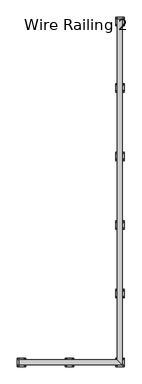
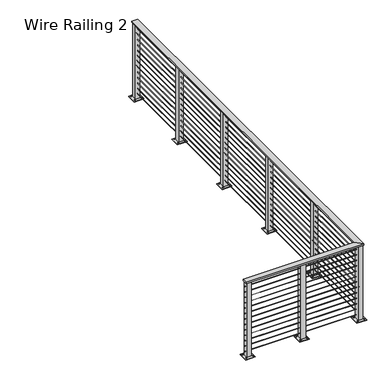
"""IFC4 building model written with IfcOpenShell, lengths in millimetres: railing geometry, Wire Railing 2."""

from ifc_helpers import new_model, si_unit, point, frame, frame_2d, origin, place, context, project, spatial, polyline, circle_curve, ellipse_curve, trimmed, segment, composite_curve, outline, extrude, faceted_brep, source, transform, mapped, element, save
from ifc_brep_helpers import plane_surface, cylinder_surface, advanced_brep


def wire_railing_2_7f4d2c74(model_context):
    return source(origin(), model_context, "Body", "SolidModel", [
        faceted_brep([(21482.8370052, 7634.1103648, 3870.325), (21559.0370052, 7634.1103648, 3870.325), (21559.0370052, 7634.1103648, 3851.275), (21482.8370052, 7634.1103648, 3851.275), (21559.0370052, 2430.2853648, 3870.325), (21559.0370052, 2430.2853648, 3851.275), (21482.8370052, 2506.4853648, 3870.325), (20003.2870052, 2506.4853648, 3870.325), (20003.2870052, 2506.4853648, 3851.275), (20003.2870052, 2430.2853648, 3851.275), (20003.2870052, 2430.2853648, 3870.325), (21482.8370052, 2506.4853648, 3851.275)], [[[0, 1, 2, 3]], [[2, 1, 4, 5]], [[1, 0, 6, 4]], [[7, 8, 9, 10]], [[5, 4, 10, 9]], [[4, 6, 7, 10]], [[3, 2, 5, 11]], [[0, 3, 11, 6]], [[11, 5, 9, 8]], [[6, 11, 8, 7]]]),
        advanced_brep(
        [(21523.3182552, 7634.1103648, 3791.74375), (21518.5557552, 7634.1103648, 3791.74375), (20003.2870052, 2466.0041148, 3791.74375), (20003.2870052, 2470.7666148, 3791.74375), (21523.3182552, 2466.0041148, 3791.74375), (21518.5557552, 2470.7666148, 3791.74375)],
        [
            (0, 1, circle_curve(frame((21520.9370052, 7634.1103648, 3791.74375), z_axis=(0.0, 1.0, 0.0), x_axis=(-1.0, 0.0, 0.0)), 2.38125)),
            (1, 0, circle_curve(frame((21520.9370052, 7634.1103648, 3791.74375), z_axis=(0.0, 1.0, 0.0), x_axis=(-1.0, 0.0, 0.0)), 2.38125)),
            (2, 3, circle_curve(frame((20003.2870052, 2468.3853648, 3791.74375), z_axis=(-1.0, 0.0, 0.0), x_axis=(0.0, 1.0, 0.0)), 2.38125)),
            (3, 2, circle_curve(frame((20003.2870052, 2468.3853648, 3791.74375), z_axis=(-1.0, 0.0, 0.0), x_axis=(0.0, 1.0, 0.0)), 2.38125)),
            (0, 4),
            (4, 5, ellipse_curve(frame((21520.9370052, 2468.3853648, 3791.74375), z_axis=(0.7071067811865475, 0.7071067811865475, 0.0), x_axis=(-0.7071067811865474, 0.7071067811865476, 0.0)), 3.367596, 2.38125)),
            (5, 1),
            (5, 4, ellipse_curve(frame((21520.9370052, 2468.3853648, 3791.74375), z_axis=(0.7071067811865475, 0.7071067811865475, 0.0), x_axis=(-0.7071067811865474, 0.7071067811865476, 0.0)), 3.367596, 2.38125)),
            (4, 2),
            (3, 5),
        ],
        [
            plane_surface(frame((21520.9370052, 7634.1103648, 3794.125), z_axis=(0.0, 1.0, 0.0), x_axis=(0.0, 0.0, -1.0))),
            plane_surface(frame((20003.2870052, 2468.3853648, 3794.125), z_axis=(-1.0, 0.0, 0.0), x_axis=(0.0, -1.0, 0.0))),
            cylinder_surface(frame((21520.9370052, 7634.1103648, 3791.74375), z_axis=(0.0, 1.0, 0.0), x_axis=(-1.0, 0.0, 0.0)), 2.38125),
            cylinder_surface(frame((21520.9370052, 2468.3853648, 3791.74375), z_axis=(1.0, 0.0, 0.0), x_axis=(0.0, 1.0, 0.0)), 2.38125),
        ],
        [
            (0, [[1, 2]]),
            (1, [[3, 4]]),
            (2, [[-1, 5, 6, 7]]),
            (2, [[-2, -7, 8, -5]]),
            (3, [[-6, 9, -4, 10]]),
            (3, [[-8, -10, -3, -9]]),
        ],
    ),
        advanced_brep(
        [(21523.3182552, 7634.1103648, 3715.54375), (21518.5557552, 7634.1103648, 3715.54375), (21523.3182552, 2466.0041148, 3715.54375), (21518.5557552, 2470.7666148, 3715.54375), (20003.2870052, 2466.0041148, 3715.54375), (20003.2870052, 2470.7666148, 3715.54375)],
        [
            (0, 1, circle_curve(frame((21520.9370052, 7634.1103648, 3715.54375), z_axis=(0.0, 1.0, 0.0), x_axis=(-1.0, 0.0, 0.0)), 2.38125)),
            (1, 0, circle_curve(frame((21520.9370052, 7634.1103648, 3715.54375), z_axis=(0.0, 1.0, 0.0), x_axis=(-1.0, 0.0, 0.0)), 2.38125)),
            (0, 2),
            (2, 3, ellipse_curve(frame((21520.9370052, 2468.3853648, 3715.54375), z_axis=(0.7071067811865475, 0.7071067811865475, 0.0), x_axis=(-0.7071067811865474, 0.7071067811865476, 0.0)), 3.367596, 2.38125)),
            (3, 1),
            (3, 2, ellipse_curve(frame((21520.9370052, 2468.3853648, 3715.54375), z_axis=(0.7071067811865475, 0.7071067811865475, 0.0), x_axis=(-0.7071067811865474, 0.7071067811865476, 0.0)), 3.367596, 2.38125)),
            (4, 5, circle_curve(frame((20003.2870052, 2468.3853648, 3715.54375), z_axis=(-1.0, 0.0, 0.0), x_axis=(0.0, 1.0, 0.0)), 2.38125)),
            (5, 4, circle_curve(frame((20003.2870052, 2468.3853648, 3715.54375), z_axis=(-1.0, 0.0, 0.0), x_axis=(0.0, 1.0, 0.0)), 2.38125)),
            (2, 4),
            (5, 3),
        ],
        [
            plane_surface(frame((21520.9370052, 7634.1103648, 3717.925), z_axis=(0.0, 1.0, 0.0), x_axis=(0.0, 0.0, -1.0))),
            cylinder_surface(frame((21520.9370052, 7634.1103648, 3715.54375), z_axis=(0.0, 1.0, 0.0), x_axis=(-1.0, 0.0, 0.0)), 2.38125),
            plane_surface(frame((20003.2870052, 2468.3853648, 3717.925), z_axis=(-1.0, 0.0, 0.0), x_axis=(0.0, -1.0, 0.0))),
            cylinder_surface(frame((21520.9370052, 2468.3853648, 3715.54375), z_axis=(1.0, 0.0, 0.0), x_axis=(0.0, 1.0, 0.0)), 2.38125),
        ],
        [
            (0, [[1, 2]]),
            (1, [[-1, 3, 4, 5]]),
            (1, [[-2, -5, 6, -3]]),
            (2, [[7, 8]]),
            (3, [[-4, 9, -8, 10]]),
            (3, [[-6, -10, -7, -9]]),
        ],
    ),
        advanced_brep(
        [(21523.3182552, 7634.1103648, 3639.34375), (21518.5557552, 7634.1103648, 3639.34375), (21523.3182552, 2466.0041148, 3639.34375), (21518.5557552, 2470.7666148, 3639.34375), (20003.2870052, 2466.0041148, 3639.34375), (20003.2870052, 2470.7666148, 3639.34375)],
        [
            (0, 1, circle_curve(frame((21520.9370052, 7634.1103648, 3639.34375), z_axis=(0.0, 1.0, 0.0), x_axis=(-1.0, 0.0, 0.0)), 2.38125)),
            (1, 0, circle_curve(frame((21520.9370052, 7634.1103648, 3639.34375), z_axis=(0.0, 1.0, 0.0), x_axis=(-1.0, 0.0, 0.0)), 2.38125)),
            (0, 2),
            (2, 3, ellipse_curve(frame((21520.9370052, 2468.3853648, 3639.34375), z_axis=(0.7071067811865475, 0.7071067811865475, 0.0), x_axis=(-0.7071067811865474, 0.7071067811865476, 0.0)), 3.367596, 2.38125)),
            (3, 1),
            (3, 2, ellipse_curve(frame((21520.9370052, 2468.3853648, 3639.34375), z_axis=(0.7071067811865475, 0.7071067811865475, 0.0), x_axis=(-0.7071067811865474, 0.7071067811865476, 0.0)), 3.367596, 2.38125)),
            (4, 5, circle_curve(frame((20003.2870052, 2468.3853648, 3639.34375), z_axis=(-1.0, 0.0, 0.0), x_axis=(0.0, 1.0, 0.0)), 2.38125)),
            (5, 4, circle_curve(frame((20003.2870052, 2468.3853648, 3639.34375), z_axis=(-1.0, 0.0, 0.0), x_axis=(0.0, 1.0, 0.0)), 2.38125)),
            (2, 4),
            (5, 3),
        ],
        [
            plane_surface(frame((21520.9370052, 7634.1103648, 3641.725), z_axis=(0.0, 1.0, 0.0), x_axis=(0.0, 0.0, -1.0))),
            cylinder_surface(frame((21520.9370052, 7634.1103648, 3639.34375), z_axis=(0.0, 1.0, 0.0), x_axis=(-1.0, 0.0, 0.0)), 2.38125),
            plane_surface(frame((20003.2870052, 2468.3853648, 3641.725), z_axis=(-1.0, 0.0, 0.0), x_axis=(0.0, -1.0, 0.0))),
            cylinder_surface(frame((21520.9370052, 2468.3853648, 3639.34375), z_axis=(1.0, 0.0, 0.0), x_axis=(0.0, 1.0, 0.0)), 2.38125),
        ],
        [
            (0, [[1, 2]]),
            (1, [[-1, 3, 4, 5]]),
            (1, [[-2, -5, 6, -3]]),
            (2, [[7, 8]]),
            (3, [[-4, 9, -8, 10]]),
            (3, [[-6, -10, -7, -9]]),
        ],
    ),
        advanced_brep(
        [(21523.3182552, 7634.1103648, 3563.14375), (21518.5557552, 7634.1103648, 3563.14375), (21523.3182552, 2466.0041148, 3563.14375), (21518.5557552, 2470.7666148, 3563.14375), (20003.2870052, 2466.0041148, 3563.14375), (20003.2870052, 2470.7666148, 3563.14375)],
        [
            (0, 1, circle_curve(frame((21520.9370052, 7634.1103648, 3563.14375), z_axis=(0.0, 1.0, 0.0), x_axis=(-1.0, 0.0, 0.0)), 2.38125)),
            (1, 0, circle_curve(frame((21520.9370052, 7634.1103648, 3563.14375), z_axis=(0.0, 1.0, 0.0), x_axis=(-1.0, 0.0, 0.0)), 2.38125)),
            (0, 2),
            (2, 3, ellipse_curve(frame((21520.9370052, 2468.3853648, 3563.14375), z_axis=(0.7071067811865475, 0.7071067811865475, 0.0), x_axis=(-0.7071067811865474, 0.7071067811865476, 0.0)), 3.367596, 2.38125)),
            (3, 1),
            (3, 2, ellipse_curve(frame((21520.9370052, 2468.3853648, 3563.14375), z_axis=(0.7071067811865475, 0.7071067811865475, 0.0), x_axis=(-0.7071067811865474, 0.7071067811865476, 0.0)), 3.367596, 2.38125)),
            (4, 5, circle_curve(frame((20003.2870052, 2468.3853648, 3563.14375), z_axis=(-1.0, 0.0, 0.0), x_axis=(0.0, 1.0, 0.0)), 2.38125)),
            (5, 4, circle_curve(frame((20003.2870052, 2468.3853648, 3563.14375), z_axis=(-1.0, 0.0, 0.0), x_axis=(0.0, 1.0, 0.0)), 2.38125)),
            (2, 4),
            (5, 3),
        ],
        [
            plane_surface(frame((21520.9370052, 7634.1103648, 3565.525), z_axis=(0.0, 1.0, 0.0), x_axis=(0.0, 0.0, -1.0))),
            cylinder_surface(frame((21520.9370052, 7634.1103648, 3563.14375), z_axis=(0.0, 1.0, 0.0), x_axis=(-1.0, 0.0, 0.0)), 2.38125),
            plane_surface(frame((20003.2870052, 2468.3853648, 3565.525), z_axis=(-1.0, 0.0, 0.0), x_axis=(0.0, -1.0, 0.0))),
            cylinder_surface(frame((21520.9370052, 2468.3853648, 3563.14375), z_axis=(1.0, 0.0, 0.0), x_axis=(0.0, 1.0, 0.0)), 2.38125),
        ],
        [
            (0, [[1, 2]]),
            (1, [[-1, 3, 4, 5]]),
            (1, [[-2, -5, 6, -3]]),
            (2, [[7, 8]]),
            (3, [[-4, 9, -8, 10]]),
            (3, [[-6, -10, -7, -9]]),
        ],
    ),
        advanced_brep(
        [(21523.3182552, 7634.1103648, 3486.94375), (21518.5557552, 7634.1103648, 3486.94375), (21523.3182552, 2466.0041148, 3486.94375), (21518.5557552, 2470.7666148, 3486.94375), (20003.2870052, 2466.0041148, 3486.94375), (20003.2870052, 2470.7666148, 3486.94375)],
        [
            (0, 1, circle_curve(frame((21520.9370052, 7634.1103648, 3486.94375), z_axis=(0.0, 1.0, 0.0), x_axis=(-1.0, 0.0, 0.0)), 2.38125)),
            (1, 0, circle_curve(frame((21520.9370052, 7634.1103648, 3486.94375), z_axis=(0.0, 1.0, 0.0), x_axis=(-1.0, 0.0, 0.0)), 2.38125)),
            (0, 2),
            (2, 3, ellipse_curve(frame((21520.9370052, 2468.3853648, 3486.94375), z_axis=(0.7071067811865475, 0.7071067811865475, 0.0), x_axis=(-0.7071067811865474, 0.7071067811865476, 0.0)), 3.367596, 2.38125)),
            (3, 1),
            (3, 2, ellipse_curve(frame((21520.9370052, 2468.3853648, 3486.94375), z_axis=(0.7071067811865475, 0.7071067811865475, 0.0), x_axis=(-0.7071067811865474, 0.7071067811865476, 0.0)), 3.367596, 2.38125)),
            (4, 5, circle_curve(frame((20003.2870052, 2468.3853648, 3486.94375), z_axis=(-1.0, 0.0, 0.0), x_axis=(0.0, 1.0, 0.0)), 2.38125)),
            (5, 4, circle_curve(frame((20003.2870052, 2468.3853648, 3486.94375), z_axis=(-1.0, 0.0, 0.0), x_axis=(0.0, 1.0, 0.0)), 2.38125)),
            (2, 4),
            (5, 3),
        ],
        [
            plane_surface(frame((21520.9370052, 7634.1103648, 3489.325), z_axis=(0.0, 1.0, 0.0), x_axis=(0.0, 0.0, -1.0))),
            cylinder_surface(frame((21520.9370052, 7634.1103648, 3486.94375), z_axis=(0.0, 1.0, 0.0), x_axis=(-1.0, 0.0, 0.0)), 2.38125),
            plane_surface(frame((20003.2870052, 2468.3853648, 3489.325), z_axis=(-1.0, 0.0, 0.0), x_axis=(0.0, -1.0, 0.0))),
            cylinder_surface(frame((21520.9370052, 2468.3853648, 3486.94375), z_axis=(1.0, 0.0, 0.0), x_axis=(0.0, 1.0, 0.0)), 2.38125),
        ],
        [
            (0, [[1, 2]]),
            (1, [[-1, 3, 4, 5]]),
            (1, [[-2, -5, 6, -3]]),
            (2, [[7, 8]]),
            (3, [[-4, 9, -8, 10]]),
            (3, [[-6, -10, -7, -9]]),
        ],
    ),
        advanced_brep(
        [(21523.3182552, 7634.1103648, 3410.74375), (21518.5557552, 7634.1103648, 3410.74375), (21523.3182552, 2466.0041148, 3410.74375), (21518.5557552, 2470.7666148, 3410.74375), (20003.2870052, 2466.0041148, 3410.74375), (20003.2870052, 2470.7666148, 3410.74375)],
        [
            (0, 1, circle_curve(frame((21520.9370052, 7634.1103648, 3410.74375), z_axis=(0.0, 1.0, 0.0), x_axis=(-1.0, 0.0, 0.0)), 2.38125)),
            (1, 0, circle_curve(frame((21520.9370052, 7634.1103648, 3410.74375), z_axis=(0.0, 1.0, 0.0), x_axis=(-1.0, 0.0, 0.0)), 2.38125)),
            (0, 2),
            (2, 3, ellipse_curve(frame((21520.9370052, 2468.3853648, 3410.74375), z_axis=(0.7071067811865475, 0.7071067811865475, 0.0), x_axis=(-0.7071067811865474, 0.7071067811865476, 0.0)), 3.367596, 2.38125)),
            (3, 1),
            (3, 2, ellipse_curve(frame((21520.9370052, 2468.3853648, 3410.74375), z_axis=(0.7071067811865475, 0.7071067811865475, 0.0), x_axis=(-0.7071067811865474, 0.7071067811865476, 0.0)), 3.367596, 2.38125)),
            (4, 5, circle_curve(frame((20003.2870052, 2468.3853648, 3410.74375), z_axis=(-1.0, 0.0, 0.0), x_axis=(0.0, 1.0, 0.0)), 2.38125)),
            (5, 4, circle_curve(frame((20003.2870052, 2468.3853648, 3410.74375), z_axis=(-1.0, 0.0, 0.0), x_axis=(0.0, 1.0, 0.0)), 2.38125)),
            (2, 4),
            (5, 3),
        ],
        [
            plane_surface(frame((21520.9370052, 7634.1103648, 3413.125), z_axis=(0.0, 1.0, 0.0), x_axis=(0.0, 0.0, -1.0))),
            cylinder_surface(frame((21520.9370052, 7634.1103648, 3410.74375), z_axis=(0.0, 1.0, 0.0), x_axis=(-1.0, 0.0, 0.0)), 2.38125),
            plane_surface(frame((20003.2870052, 2468.3853648, 3413.125), z_axis=(-1.0, 0.0, 0.0), x_axis=(0.0, -1.0, 0.0))),
            cylinder_surface(frame((21520.9370052, 2468.3853648, 3410.74375), z_axis=(1.0, 0.0, 0.0), x_axis=(0.0, 1.0, 0.0)), 2.38125),
        ],
        [
            (0, [[1, 2]]),
            (1, [[-1, 3, 4, 5]]),
            (1, [[-2, -5, 6, -3]]),
            (2, [[7, 8]]),
            (3, [[-4, 9, -8, 10]]),
            (3, [[-6, -10, -7, -9]]),
        ],
    ),
        advanced_brep(
        [(21523.3182552, 7634.1103648, 3334.54375), (21518.5557552, 7634.1103648, 3334.54375), (21523.3182552, 2466.0041148, 3334.54375), (21518.5557552, 2470.7666148, 3334.54375), (20003.2870052, 2466.0041148, 3334.54375), (20003.2870052, 2470.7666148, 3334.54375)],
        [
            (0, 1, circle_curve(frame((21520.9370052, 7634.1103648, 3334.54375), z_axis=(0.0, 1.0, 0.0), x_axis=(-1.0, 0.0, 0.0)), 2.38125)),
            (1, 0, circle_curve(frame((21520.9370052, 7634.1103648, 3334.54375), z_axis=(0.0, 1.0, 0.0), x_axis=(-1.0, 0.0, 0.0)), 2.38125)),
            (0, 2),
            (2, 3, ellipse_curve(frame((21520.9370052, 2468.3853648, 3334.54375), z_axis=(0.7071067811865475, 0.7071067811865475, 0.0), x_axis=(-0.7071067811865474, 0.7071067811865476, 0.0)), 3.367596, 2.38125)),
            (3, 1),
            (3, 2, ellipse_curve(frame((21520.9370052, 2468.3853648, 3334.54375), z_axis=(0.7071067811865475, 0.7071067811865475, 0.0), x_axis=(-0.7071067811865474, 0.7071067811865476, 0.0)), 3.367596, 2.38125)),
            (4, 5, circle_curve(frame((20003.2870052, 2468.3853648, 3334.54375), z_axis=(-1.0, 0.0, 0.0), x_axis=(0.0, 1.0, 0.0)), 2.38125)),
            (5, 4, circle_curve(frame((20003.2870052, 2468.3853648, 3334.54375), z_axis=(-1.0, 0.0, 0.0), x_axis=(0.0, 1.0, 0.0)), 2.38125)),
            (2, 4),
            (5, 3),
        ],
        [
            plane_surface(frame((21520.9370052, 7634.1103648, 3336.925), z_axis=(0.0, 1.0, 0.0), x_axis=(0.0, 0.0, -1.0))),
            cylinder_surface(frame((21520.9370052, 7634.1103648, 3334.54375), z_axis=(0.0, 1.0, 0.0), x_axis=(-1.0, 0.0, 0.0)), 2.38125),
            plane_surface(frame((20003.2870052, 2468.3853648, 3336.925), z_axis=(-1.0, 0.0, 0.0), x_axis=(0.0, -1.0, 0.0))),
            cylinder_surface(frame((21520.9370052, 2468.3853648, 3334.54375), z_axis=(1.0, 0.0, 0.0), x_axis=(0.0, 1.0, 0.0)), 2.38125),
        ],
        [
            (0, [[1, 2]]),
            (1, [[-1, 3, 4, 5]]),
            (1, [[-2, -5, 6, -3]]),
            (2, [[7, 8]]),
            (3, [[-4, 9, -8, 10]]),
            (3, [[-6, -10, -7, -9]]),
        ],
    ),
        advanced_brep(
        [(21523.3182552, 7634.1103648, 3258.34375), (21518.5557552, 7634.1103648, 3258.34375), (21523.3182552, 2466.0041148, 3258.34375), (21518.5557552, 2470.7666148, 3258.34375), (20003.2870052, 2466.0041148, 3258.34375), (20003.2870052, 2470.7666148, 3258.34375)],
        [
            (0, 1, circle_curve(frame((21520.9370052, 7634.1103648, 3258.34375), z_axis=(0.0, 1.0, 0.0), x_axis=(-1.0, 0.0, 0.0)), 2.38125)),
            (1, 0, circle_curve(frame((21520.9370052, 7634.1103648, 3258.34375), z_axis=(0.0, 1.0, 0.0), x_axis=(-1.0, 0.0, 0.0)), 2.38125)),
            (0, 2),
            (2, 3, ellipse_curve(frame((21520.9370052, 2468.3853648, 3258.34375), z_axis=(0.7071067811865475, 0.7071067811865475, 0.0), x_axis=(-0.7071067811865474, 0.7071067811865476, 0.0)), 3.367596, 2.38125)),
            (3, 1),
            (3, 2, ellipse_curve(frame((21520.9370052, 2468.3853648, 3258.34375), z_axis=(0.7071067811865475, 0.7071067811865475, 0.0), x_axis=(-0.7071067811865474, 0.7071067811865476, 0.0)), 3.367596, 2.38125)),
            (4, 5, circle_curve(frame((20003.2870052, 2468.3853648, 3258.34375), z_axis=(-1.0, 0.0, 0.0), x_axis=(0.0, 1.0, 0.0)), 2.38125)),
            (5, 4, circle_curve(frame((20003.2870052, 2468.3853648, 3258.34375), z_axis=(-1.0, 0.0, 0.0), x_axis=(0.0, 1.0, 0.0)), 2.38125)),
            (2, 4),
            (5, 3),
        ],
        [
            plane_surface(frame((21520.9370052, 7634.1103648, 3260.725), z_axis=(0.0, 1.0, 0.0), x_axis=(0.0, 0.0, -1.0))),
            cylinder_surface(frame((21520.9370052, 7634.1103648, 3258.34375), z_axis=(0.0, 1.0, 0.0), x_axis=(-1.0, 0.0, 0.0)), 2.38125),
            plane_surface(frame((20003.2870052, 2468.3853648, 3260.725), z_axis=(-1.0, 0.0, 0.0), x_axis=(0.0, -1.0, 0.0))),
            cylinder_surface(frame((21520.9370052, 2468.3853648, 3258.34375), z_axis=(1.0, 0.0, 0.0), x_axis=(0.0, 1.0, 0.0)), 2.38125),
        ],
        [
            (0, [[1, 2]]),
            (1, [[-1, 3, 4, 5]]),
            (1, [[-2, -5, 6, -3]]),
            (2, [[7, 8]]),
            (3, [[-4, 9, -8, 10]]),
            (3, [[-6, -10, -7, -9]]),
        ],
    ),
        advanced_brep(
        [(21523.3182552, 7634.1103648, 3182.14375), (21518.5557552, 7634.1103648, 3182.14375), (21523.3182552, 2466.0041148, 3182.14375), (21518.5557552, 2470.7666148, 3182.14375), (20003.2870052, 2466.0041148, 3182.14375), (20003.2870052, 2470.7666148, 3182.14375)],
        [
            (0, 1, circle_curve(frame((21520.9370052, 7634.1103648, 3182.14375), z_axis=(0.0, 1.0, 0.0), x_axis=(-1.0, 0.0, 0.0)), 2.38125)),
            (1, 0, circle_curve(frame((21520.9370052, 7634.1103648, 3182.14375), z_axis=(0.0, 1.0, 0.0), x_axis=(-1.0, 0.0, 0.0)), 2.38125)),
            (0, 2),
            (2, 3, ellipse_curve(frame((21520.9370052, 2468.3853648, 3182.14375), z_axis=(0.7071067811865475, 0.7071067811865475, 0.0), x_axis=(-0.7071067811865474, 0.7071067811865476, 0.0)), 3.367596, 2.38125)),
            (3, 1),
            (3, 2, ellipse_curve(frame((21520.9370052, 2468.3853648, 3182.14375), z_axis=(0.7071067811865475, 0.7071067811865475, 0.0), x_axis=(-0.7071067811865474, 0.7071067811865476, 0.0)), 3.367596, 2.38125)),
            (4, 5, circle_curve(frame((20003.2870052, 2468.3853648, 3182.14375), z_axis=(-1.0, 0.0, 0.0), x_axis=(0.0, 1.0, 0.0)), 2.38125)),
            (5, 4, circle_curve(frame((20003.2870052, 2468.3853648, 3182.14375), z_axis=(-1.0, 0.0, 0.0), x_axis=(0.0, 1.0, 0.0)), 2.38125)),
            (2, 4),
            (5, 3),
        ],
        [
            plane_surface(frame((21520.9370052, 7634.1103648, 3184.525), z_axis=(0.0, 1.0, 0.0), x_axis=(0.0, 0.0, -1.0))),
            cylinder_surface(frame((21520.9370052, 7634.1103648, 3182.14375), z_axis=(0.0, 1.0, 0.0), x_axis=(-1.0, 0.0, 0.0)), 2.38125),
            plane_surface(frame((20003.2870052, 2468.3853648, 3184.525), z_axis=(-1.0, 0.0, 0.0), x_axis=(0.0, -1.0, 0.0))),
            cylinder_surface(frame((21520.9370052, 2468.3853648, 3182.14375), z_axis=(1.0, 0.0, 0.0), x_axis=(0.0, 1.0, 0.0)), 2.38125),
        ],
        [
            (0, [[1, 2]]),
            (1, [[-1, 3, 4, 5]]),
            (1, [[-2, -5, 6, -3]]),
            (2, [[7, 8]]),
            (3, [[-4, 9, -8, 10]]),
            (3, [[-6, -10, -7, -9]]),
        ],
    ),
        advanced_brep(
        [(21523.3182552, 7634.1103648, 3105.94375), (21518.5557552, 7634.1103648, 3105.94375), (21523.3182552, 2466.0041148, 3105.94375), (21518.5557552, 2470.7666148, 3105.94375), (20003.2870052, 2466.0041148, 3105.94375), (20003.2870052, 2470.7666148, 3105.94375)],
        [
            (0, 1, circle_curve(frame((21520.9370052, 7634.1103648, 3105.94375), z_axis=(0.0, 1.0, 0.0), x_axis=(-1.0, 0.0, 0.0)), 2.38125)),
            (1, 0, circle_curve(frame((21520.9370052, 7634.1103648, 3105.94375), z_axis=(0.0, 1.0, 0.0), x_axis=(-1.0, 0.0, 0.0)), 2.38125)),
            (0, 2),
            (2, 3, ellipse_curve(frame((21520.9370052, 2468.3853648, 3105.94375), z_axis=(0.7071067811865475, 0.7071067811865475, 0.0), x_axis=(-0.7071067811865474, 0.7071067811865476, 0.0)), 3.367596, 2.38125)),
            (3, 1),
            (3, 2, ellipse_curve(frame((21520.9370052, 2468.3853648, 3105.94375), z_axis=(0.7071067811865475, 0.7071067811865475, 0.0), x_axis=(-0.7071067811865474, 0.7071067811865476, 0.0)), 3.367596, 2.38125)),
            (4, 5, circle_curve(frame((20003.2870052, 2468.3853648, 3105.94375), z_axis=(-1.0, 0.0, 0.0), x_axis=(0.0, 1.0, 0.0)), 2.38125)),
            (5, 4, circle_curve(frame((20003.2870052, 2468.3853648, 3105.94375), z_axis=(-1.0, 0.0, 0.0), x_axis=(0.0, 1.0, 0.0)), 2.38125)),
            (2, 4),
            (5, 3),
        ],
        [
            plane_surface(frame((21520.9370052, 7634.1103648, 3108.325), z_axis=(0.0, 1.0, 0.0), x_axis=(0.0, 0.0, -1.0))),
            cylinder_surface(frame((21520.9370052, 7634.1103648, 3105.94375), z_axis=(0.0, 1.0, 0.0), x_axis=(-1.0, 0.0, 0.0)), 2.38125),
            plane_surface(frame((20003.2870052, 2468.3853648, 3108.325), z_axis=(-1.0, 0.0, 0.0), x_axis=(0.0, -1.0, 0.0))),
            cylinder_surface(frame((21520.9370052, 2468.3853648, 3105.94375), z_axis=(1.0, 0.0, 0.0), x_axis=(0.0, 1.0, 0.0)), 2.38125),
        ],
        [
            (0, [[1, 2]]),
            (1, [[-1, 3, 4, 5]]),
            (1, [[-2, -5, 6, -3]]),
            (2, [[7, 8]]),
            (3, [[-4, 9, -8, 10]]),
            (3, [[-6, -10, -7, -9]]),
        ],
    ),
        advanced_brep(
        [(21523.3182552, 7634.1103648, 3029.74375), (21518.5557552, 7634.1103648, 3029.74375), (21523.3182552, 2466.0041148, 3029.74375), (21518.5557552, 2470.7666148, 3029.74375), (20003.2870052, 2466.0041148, 3029.74375), (20003.2870052, 2470.7666148, 3029.74375)],
        [
            (0, 1, circle_curve(frame((21520.9370052, 7634.1103648, 3029.74375), z_axis=(0.0, 1.0, 0.0), x_axis=(-1.0, 0.0, 0.0)), 2.38125)),
            (1, 0, circle_curve(frame((21520.9370052, 7634.1103648, 3029.74375), z_axis=(0.0, 1.0, 0.0), x_axis=(-1.0, 0.0, 0.0)), 2.38125)),
            (0, 2),
            (2, 3, ellipse_curve(frame((21520.9370052, 2468.3853648, 3029.74375), z_axis=(0.7071067811865475, 0.7071067811865475, 0.0), x_axis=(-0.7071067811865474, 0.7071067811865476, 0.0)), 3.367596, 2.38125)),
            (3, 1),
            (3, 2, ellipse_curve(frame((21520.9370052, 2468.3853648, 3029.74375), z_axis=(0.7071067811865475, 0.7071067811865475, 0.0), x_axis=(-0.7071067811865474, 0.7071067811865476, 0.0)), 3.367596, 2.38125)),
            (4, 5, circle_curve(frame((20003.2870052, 2468.3853648, 3029.74375), z_axis=(-1.0, 0.0, 0.0), x_axis=(0.0, 1.0, 0.0)), 2.38125)),
            (5, 4, circle_curve(frame((20003.2870052, 2468.3853648, 3029.74375), z_axis=(-1.0, 0.0, 0.0), x_axis=(0.0, 1.0, 0.0)), 2.38125)),
            (2, 4),
            (5, 3),
        ],
        [
            plane_surface(frame((21520.9370052, 7634.1103648, 3032.125), z_axis=(0.0, 1.0, 0.0), x_axis=(0.0, 0.0, -1.0))),
            cylinder_surface(frame((21520.9370052, 7634.1103648, 3029.74375), z_axis=(0.0, 1.0, 0.0), x_axis=(-1.0, 0.0, 0.0)), 2.38125),
            plane_surface(frame((20003.2870052, 2468.3853648, 3032.125), z_axis=(-1.0, 0.0, 0.0), x_axis=(0.0, -1.0, 0.0))),
            cylinder_surface(frame((21520.9370052, 2468.3853648, 3029.74375), z_axis=(1.0, 0.0, 0.0), x_axis=(0.0, 1.0, 0.0)), 2.38125),
        ],
        [
            (0, [[1, 2]]),
            (1, [[-1, 3, 4, 5]]),
            (1, [[-2, -5, 6, -3]]),
            (2, [[7, 8]]),
            (3, [[-4, 9, -8, 10]]),
            (3, [[-6, -10, -7, -9]]),
        ],
    ),
        advanced_brep(
        [(21523.3182552, 7634.1103648, 2953.54375), (21518.5557552, 7634.1103648, 2953.54375), (21523.3182552, 2466.0041148, 2953.54375), (21518.5557552, 2470.7666148, 2953.54375), (20003.2870052, 2466.0041148, 2953.54375), (20003.2870052, 2470.7666148, 2953.54375)],
        [
            (0, 1, circle_curve(frame((21520.9370052, 7634.1103648, 2953.54375), z_axis=(0.0, 1.0, 0.0), x_axis=(-1.0, 0.0, 0.0)), 2.38125)),
            (1, 0, circle_curve(frame((21520.9370052, 7634.1103648, 2953.54375), z_axis=(0.0, 1.0, 0.0), x_axis=(-1.0, 0.0, 0.0)), 2.38125)),
            (0, 2),
            (2, 3, ellipse_curve(frame((21520.9370052, 2468.3853648, 2953.54375), z_axis=(0.7071067811865475, 0.7071067811865475, 0.0), x_axis=(-0.7071067811865474, 0.7071067811865476, 0.0)), 3.367596, 2.38125)),
            (3, 1),
            (3, 2, ellipse_curve(frame((21520.9370052, 2468.3853648, 2953.54375), z_axis=(0.7071067811865475, 0.7071067811865475, 0.0), x_axis=(-0.7071067811865474, 0.7071067811865476, 0.0)), 3.367596, 2.38125)),
            (4, 5, circle_curve(frame((20003.2870052, 2468.3853648, 2953.54375), z_axis=(-1.0, 0.0, 0.0), x_axis=(0.0, 1.0, 0.0)), 2.38125)),
            (5, 4, circle_curve(frame((20003.2870052, 2468.3853648, 2953.54375), z_axis=(-1.0, 0.0, 0.0), x_axis=(0.0, 1.0, 0.0)), 2.38125)),
            (2, 4),
            (5, 3),
        ],
        [
            plane_surface(frame((21520.9370052, 7634.1103648, 2955.925), z_axis=(0.0, 1.0, 0.0), x_axis=(0.0, 0.0, -1.0))),
            cylinder_surface(frame((21520.9370052, 7634.1103648, 2953.54375), z_axis=(0.0, 1.0, 0.0), x_axis=(-1.0, 0.0, 0.0)), 2.38125),
            plane_surface(frame((20003.2870052, 2468.3853648, 2955.925), z_axis=(-1.0, 0.0, 0.0), x_axis=(0.0, -1.0, 0.0))),
            cylinder_surface(frame((21520.9370052, 2468.3853648, 2953.54375), z_axis=(1.0, 0.0, 0.0), x_axis=(0.0, 1.0, 0.0)), 2.38125),
        ],
        [
            (0, [[1, 2]]),
            (1, [[-1, 3, 4, 5]]),
            (1, [[-2, -5, 6, -3]]),
            (2, [[7, 8]]),
            (3, [[-4, 9, -8, 10]]),
            (3, [[-6, -10, -7, -9]]),
        ],
    ),
        advanced_brep(
        [(21523.3182552, 7634.1103648, 2877.34375), (21518.5557552, 7634.1103648, 2877.34375), (21523.3182552, 2466.0041148, 2877.34375), (21518.5557552, 2470.7666148, 2877.34375), (20003.2870052, 2466.0041148, 2877.34375), (20003.2870052, 2470.7666148, 2877.34375)],
        [
            (0, 1, circle_curve(frame((21520.9370052, 7634.1103648, 2877.34375), z_axis=(0.0, 1.0, 0.0), x_axis=(-1.0, 0.0, 0.0)), 2.38125)),
            (1, 0, circle_curve(frame((21520.9370052, 7634.1103648, 2877.34375), z_axis=(0.0, 1.0, 0.0), x_axis=(-1.0, 0.0, 0.0)), 2.38125)),
            (0, 2),
            (2, 3, ellipse_curve(frame((21520.9370052, 2468.3853648, 2877.34375), z_axis=(0.7071067811865475, 0.7071067811865475, 0.0), x_axis=(-0.7071067811865474, 0.7071067811865476, 0.0)), 3.367596, 2.38125)),
            (3, 1),
            (3, 2, ellipse_curve(frame((21520.9370052, 2468.3853648, 2877.34375), z_axis=(0.7071067811865475, 0.7071067811865475, 0.0), x_axis=(-0.7071067811865474, 0.7071067811865476, 0.0)), 3.367596, 2.38125)),
            (4, 5, circle_curve(frame((20003.2870052, 2468.3853648, 2877.34375), z_axis=(-1.0, 0.0, 0.0), x_axis=(0.0, 1.0, 0.0)), 2.38125)),
            (5, 4, circle_curve(frame((20003.2870052, 2468.3853648, 2877.34375), z_axis=(-1.0, 0.0, 0.0), x_axis=(0.0, 1.0, 0.0)), 2.38125)),
            (2, 4),
            (5, 3),
        ],
        [
            plane_surface(frame((21520.9370052, 7634.1103648, 2879.725), z_axis=(0.0, 1.0, 0.0), x_axis=(0.0, 0.0, -1.0))),
            cylinder_surface(frame((21520.9370052, 7634.1103648, 2877.34375), z_axis=(0.0, 1.0, 0.0), x_axis=(-1.0, 0.0, 0.0)), 2.38125),
            plane_surface(frame((20003.2870052, 2468.3853648, 2879.725), z_axis=(-1.0, 0.0, 0.0), x_axis=(0.0, -1.0, 0.0))),
            cylinder_surface(frame((21520.9370052, 2468.3853648, 2877.34375), z_axis=(1.0, 0.0, 0.0), x_axis=(0.0, 1.0, 0.0)), 2.38125),
        ],
        [
            (0, [[1, 2]]),
            (1, [[-1, 3, 4, 5]]),
            (1, [[-2, -5, 6, -3]]),
            (2, [[7, 8]]),
            (3, [[-4, 9, -8, 10]]),
            (3, [[-6, -10, -7, -9]]),
        ],
    ),
        extrude(outline(composite_curve([segment(trimmed(circle_curve(frame_2d((20806.5620052, 2512.8353648)), 6.35), [point((20806.5620052, 2519.1853648))], [point((20806.5620052, 2506.4853648))], False, "CARTESIAN"), True, "CONTINUOUS"), segment(trimmed(circle_curve(frame_2d((20806.5620052, 2512.8353648)), 6.35), [point((20806.5620052, 2506.4853648))], [point((20806.5620052, 2519.1853648))], False, "CARTESIAN"), True, "CONTINUOUS")], self_intersect=False)), frame((0.0, 0.0, 2803.525), z_axis=(0.0, 0.0, 1.0), x_axis=(1.0, 0.0, 0.0)), (0.0, 0.0, 1.0), 12.7),
        extrude(outline(composite_curve([segment(trimmed(circle_curve(frame_2d((20806.5620052, 2423.9353648)), 6.35), [point((20806.5620052, 2430.2853648))], [point((20806.5620052, 2417.5853648))], False, "CARTESIAN"), True, "CONTINUOUS"), segment(trimmed(circle_curve(frame_2d((20806.5620052, 2423.9353648)), 6.35), [point((20806.5620052, 2417.5853648))], [point((20806.5620052, 2430.2853648))], False, "CARTESIAN"), True, "CONTINUOUS")], self_intersect=False)), frame((0.0, 0.0, 2803.525), z_axis=(0.0, 0.0, 1.0), x_axis=(1.0, 0.0, 0.0)), (0.0, 0.0, 1.0), 12.7),
        extrude(outline(composite_curve([segment(trimmed(circle_curve(frame_2d((20717.6620052, 2512.8353648)), 6.35), [point((20717.6620052, 2519.1853648))], [point((20717.6620052, 2506.4853648))], False, "CARTESIAN"), True, "CONTINUOUS"), segment(trimmed(circle_curve(frame_2d((20717.6620052, 2512.8353648)), 6.35), [point((20717.6620052, 2506.4853648))], [point((20717.6620052, 2519.1853648))], False, "CARTESIAN"), True, "CONTINUOUS")], self_intersect=False)), frame((0.0, 0.0, 2803.525), z_axis=(0.0, 0.0, 1.0), x_axis=(1.0, 0.0, 0.0)), (0.0, 0.0, 1.0), 12.7),
        extrude(outline(composite_curve([segment(trimmed(circle_curve(frame_2d((20717.6620052, 2423.9353648)), 6.35), [point((20717.6620052, 2430.2853648))], [point((20717.6620052, 2417.5853648))], False, "CARTESIAN"), True, "CONTINUOUS"), segment(trimmed(circle_curve(frame_2d((20717.6620052, 2423.9353648)), 6.35), [point((20717.6620052, 2417.5853648))], [point((20717.6620052, 2430.2853648))], False, "CARTESIAN"), True, "CONTINUOUS")], self_intersect=False)), frame((0.0, 0.0, 2803.525), z_axis=(0.0, 0.0, 1.0), x_axis=(1.0, 0.0, 0.0)), (0.0, 0.0, 1.0), 12.7),
        extrude(outline(polyline([(20825.6120052, 2404.8853648), (20698.6120052, 2404.8853648), (20698.6120052, 2531.8853648), (20825.6120052, 2531.8853648), (20825.6120052, 2404.8853648)])), frame((0.0, 0.0, 2803.525), z_axis=(0.0, 0.0, 1.0), x_axis=(1.0, 0.0, 0.0)), (0.0, 0.0, 1.0), 6.35),
        extrude(outline(polyline([(20792.2745052, 2438.2228648), (20731.9495052, 2438.2228648), (20731.9495052, 2498.5478648), (20792.2745052, 2498.5478648), (20792.2745052, 2438.2228648)]), holes=[polyline([(20785.9245052, 2444.5728648), (20785.9245052, 2492.1978648), (20738.2995052, 2492.1978648), (20738.2995052, 2444.5728648), (20785.9245052, 2444.5728648)])]), frame((0.0, 0.0, 2803.525), z_axis=(0.0, 0.0, 1.0), x_axis=(1.0, 0.0, 0.0)), (0.0, 0.0, 1.0), 1047.75),
        extrude(outline(composite_curve([segment(trimmed(circle_curve(frame_2d((21476.4870052, 3545.9803648)), 6.35), [point((21470.1370052, 3545.9803648))], [point((21482.8370052, 3545.9803648))], False, "CARTESIAN"), True, "CONTINUOUS"), segment(trimmed(circle_curve(frame_2d((21476.4870052, 3545.9803648)), 6.35), [point((21482.8370052, 3545.9803648))], [point((21470.1370052, 3545.9803648))], False, "CARTESIAN"), True, "CONTINUOUS")], self_intersect=False)), frame((0.0, 0.0, 2803.525), z_axis=(0.0, 0.0, 1.0), x_axis=(1.0, 0.0, 0.0)), (0.0, 0.0, 1.0), 12.7),
        extrude(outline(composite_curve([segment(trimmed(circle_curve(frame_2d((21565.3870052, 3545.9803648)), 6.35), [point((21559.0370052, 3545.9803648))], [point((21571.7370052, 3545.9803648))], False, "CARTESIAN"), True, "CONTINUOUS"), segment(trimmed(circle_curve(frame_2d((21565.3870052, 3545.9803648)), 6.35), [point((21571.7370052, 3545.9803648))], [point((21559.0370052, 3545.9803648))], False, "CARTESIAN"), True, "CONTINUOUS")], self_intersect=False)), frame((0.0, 0.0, 2803.525), z_axis=(0.0, 0.0, 1.0), x_axis=(1.0, 0.0, 0.0)), (0.0, 0.0, 1.0), 12.7),
        extrude(outline(composite_curve([segment(trimmed(circle_curve(frame_2d((21476.4870052, 3457.0803648)), 6.35), [point((21470.1370052, 3457.0803648))], [point((21482.8370052, 3457.0803648))], False, "CARTESIAN"), True, "CONTINUOUS"), segment(trimmed(circle_curve(frame_2d((21476.4870052, 3457.0803648)), 6.35), [point((21482.8370052, 3457.0803648))], [point((21470.1370052, 3457.0803648))], False, "CARTESIAN"), True, "CONTINUOUS")], self_intersect=False)), frame((0.0, 0.0, 2803.525), z_axis=(0.0, 0.0, 1.0), x_axis=(1.0, 0.0, 0.0)), (0.0, 0.0, 1.0), 12.7),
        extrude(outline(composite_curve([segment(trimmed(circle_curve(frame_2d((21565.3870052, 3457.0803648)), 6.35), [point((21559.0370052, 3457.0803648))], [point((21571.7370052, 3457.0803648))], False, "CARTESIAN"), True, "CONTINUOUS"), segment(trimmed(circle_curve(frame_2d((21565.3870052, 3457.0803648)), 6.35), [point((21571.7370052, 3457.0803648))], [point((21559.0370052, 3457.0803648))], False, "CARTESIAN"), True, "CONTINUOUS")], self_intersect=False)), frame((0.0, 0.0, 2803.525), z_axis=(0.0, 0.0, 1.0), x_axis=(1.0, 0.0, 0.0)), (0.0, 0.0, 1.0), 12.7),
        extrude(outline(polyline([(21584.4370052, 3565.0303648), (21584.4370052, 3438.0303648), (21457.4370052, 3438.0303648), (21457.4370052, 3565.0303648), (21584.4370052, 3565.0303648)])), frame((0.0, 0.0, 2803.525), z_axis=(0.0, 0.0, 1.0), x_axis=(1.0, 0.0, 0.0)), (0.0, 0.0, 1.0), 6.35),
        extrude(outline(polyline([(21551.0995052, 3531.6928648), (21551.0995052, 3471.3678648), (21490.7745052, 3471.3678648), (21490.7745052, 3531.6928648), (21551.0995052, 3531.6928648)]), holes=[polyline([(21544.7495052, 3525.3428648), (21497.1245052, 3525.3428648), (21497.1245052, 3477.7178648), (21544.7495052, 3477.7178648), (21544.7495052, 3525.3428648)])]), frame((0.0, 0.0, 2803.525), z_axis=(0.0, 0.0, 1.0), x_axis=(1.0, 0.0, 0.0)), (0.0, 0.0, 1.0), 1047.75),
        extrude(outline(composite_curve([segment(trimmed(circle_curve(frame_2d((21476.4870052, 4579.1253648)), 6.35), [point((21470.1370052, 4579.1253648))], [point((21482.8370052, 4579.1253648))], False, "CARTESIAN"), True, "CONTINUOUS"), segment(trimmed(circle_curve(frame_2d((21476.4870052, 4579.1253648)), 6.35), [point((21482.8370052, 4579.1253648))], [point((21470.1370052, 4579.1253648))], False, "CARTESIAN"), True, "CONTINUOUS")], self_intersect=False)), frame((0.0, 0.0, 2803.525), z_axis=(0.0, 0.0, 1.0), x_axis=(1.0, 0.0, 0.0)), (0.0, 0.0, 1.0), 12.7),
        extrude(outline(composite_curve([segment(trimmed(circle_curve(frame_2d((21565.3870052, 4579.1253648)), 6.35), [point((21559.0370052, 4579.1253648))], [point((21571.7370052, 4579.1253648))], False, "CARTESIAN"), True, "CONTINUOUS"), segment(trimmed(circle_curve(frame_2d((21565.3870052, 4579.1253648)), 6.35), [point((21571.7370052, 4579.1253648))], [point((21559.0370052, 4579.1253648))], False, "CARTESIAN"), True, "CONTINUOUS")], self_intersect=False)), frame((0.0, 0.0, 2803.525), z_axis=(0.0, 0.0, 1.0), x_axis=(1.0, 0.0, 0.0)), (0.0, 0.0, 1.0), 12.7),
        extrude(outline(composite_curve([segment(trimmed(circle_curve(frame_2d((21476.4870052, 4490.2253648)), 6.35), [point((21470.1370052, 4490.2253648))], [point((21482.8370052, 4490.2253648))], False, "CARTESIAN"), True, "CONTINUOUS"), segment(trimmed(circle_curve(frame_2d((21476.4870052, 4490.2253648)), 6.35), [point((21482.8370052, 4490.2253648))], [point((21470.1370052, 4490.2253648))], False, "CARTESIAN"), True, "CONTINUOUS")], self_intersect=False)), frame((0.0, 0.0, 2803.525), z_axis=(0.0, 0.0, 1.0), x_axis=(1.0, 0.0, 0.0)), (0.0, 0.0, 1.0), 12.7),
        extrude(outline(composite_curve([segment(trimmed(circle_curve(frame_2d((21565.3870052, 4490.2253648)), 6.35), [point((21559.0370052, 4490.2253648))], [point((21571.7370052, 4490.2253648))], False, "CARTESIAN"), True, "CONTINUOUS"), segment(trimmed(circle_curve(frame_2d((21565.3870052, 4490.2253648)), 6.35), [point((21571.7370052, 4490.2253648))], [point((21559.0370052, 4490.2253648))], False, "CARTESIAN"), True, "CONTINUOUS")], self_intersect=False)), frame((0.0, 0.0, 2803.525), z_axis=(0.0, 0.0, 1.0), x_axis=(1.0, 0.0, 0.0)), (0.0, 0.0, 1.0), 12.7),
        extrude(outline(polyline([(21584.4370052, 4598.1753648), (21584.4370052, 4471.1753648), (21457.4370052, 4471.1753648), (21457.4370052, 4598.1753648), (21584.4370052, 4598.1753648)])), frame((0.0, 0.0, 2803.525), z_axis=(0.0, 0.0, 1.0), x_axis=(1.0, 0.0, 0.0)), (0.0, 0.0, 1.0), 6.35),
        extrude(outline(polyline([(21551.0995052, 4564.8378648), (21551.0995052, 4504.5128648), (21490.7745052, 4504.5128648), (21490.7745052, 4564.8378648), (21551.0995052, 4564.8378648)]), holes=[polyline([(21544.7495052, 4558.4878648), (21497.1245052, 4558.4878648), (21497.1245052, 4510.8628648), (21544.7495052, 4510.8628648), (21544.7495052, 4558.4878648)])]), frame((0.0, 0.0, 2803.525), z_axis=(0.0, 0.0, 1.0), x_axis=(1.0, 0.0, 0.0)), (0.0, 0.0, 1.0), 1047.75),
        extrude(outline(composite_curve([segment(trimmed(circle_curve(frame_2d((21476.4870052, 5612.2703648)), 6.35), [point((21470.1370052, 5612.2703648))], [point((21482.8370052, 5612.2703648))], False, "CARTESIAN"), True, "CONTINUOUS"), segment(trimmed(circle_curve(frame_2d((21476.4870052, 5612.2703648)), 6.35), [point((21482.8370052, 5612.2703648))], [point((21470.1370052, 5612.2703648))], False, "CARTESIAN"), True, "CONTINUOUS")], self_intersect=False)), frame((0.0, 0.0, 2803.525), z_axis=(0.0, 0.0, 1.0), x_axis=(1.0, 0.0, 0.0)), (0.0, 0.0, 1.0), 12.7),
        extrude(outline(composite_curve([segment(trimmed(circle_curve(frame_2d((21565.3870052, 5612.2703648)), 6.35), [point((21559.0370052, 5612.2703648))], [point((21571.7370052, 5612.2703648))], False, "CARTESIAN"), True, "CONTINUOUS"), segment(trimmed(circle_curve(frame_2d((21565.3870052, 5612.2703648)), 6.35), [point((21571.7370052, 5612.2703648))], [point((21559.0370052, 5612.2703648))], False, "CARTESIAN"), True, "CONTINUOUS")], self_intersect=False)), frame((0.0, 0.0, 2803.525), z_axis=(0.0, 0.0, 1.0), x_axis=(1.0, 0.0, 0.0)), (0.0, 0.0, 1.0), 12.7),
        extrude(outline(composite_curve([segment(trimmed(circle_curve(frame_2d((21476.4870052, 5523.3703648)), 6.35), [point((21470.1370052, 5523.3703648))], [point((21482.8370052, 5523.3703648))], False, "CARTESIAN"), True, "CONTINUOUS"), segment(trimmed(circle_curve(frame_2d((21476.4870052, 5523.3703648)), 6.35), [point((21482.8370052, 5523.3703648))], [point((21470.1370052, 5523.3703648))], False, "CARTESIAN"), True, "CONTINUOUS")], self_intersect=False)), frame((0.0, 0.0, 2803.525), z_axis=(0.0, 0.0, 1.0), x_axis=(1.0, 0.0, 0.0)), (0.0, 0.0, 1.0), 12.7),
        extrude(outline(composite_curve([segment(trimmed(circle_curve(frame_2d((21565.3870052, 5523.3703648)), 6.35), [point((21559.0370052, 5523.3703648))], [point((21571.7370052, 5523.3703648))], False, "CARTESIAN"), True, "CONTINUOUS"), segment(trimmed(circle_curve(frame_2d((21565.3870052, 5523.3703648)), 6.35), [point((21571.7370052, 5523.3703648))], [point((21559.0370052, 5523.3703648))], False, "CARTESIAN"), True, "CONTINUOUS")], self_intersect=False)), frame((0.0, 0.0, 2803.525), z_axis=(0.0, 0.0, 1.0), x_axis=(1.0, 0.0, 0.0)), (0.0, 0.0, 1.0), 12.7),
        extrude(outline(polyline([(21584.4370052, 5631.3203648), (21584.4370052, 5504.3203648), (21457.4370052, 5504.3203648), (21457.4370052, 5631.3203648), (21584.4370052, 5631.3203648)])), frame((0.0, 0.0, 2803.525), z_axis=(0.0, 0.0, 1.0), x_axis=(1.0, 0.0, 0.0)), (0.0, 0.0, 1.0), 6.35),
        extrude(outline(polyline([(21551.0995052, 5597.9828648), (21551.0995052, 5537.6578648), (21490.7745052, 5537.6578648), (21490.7745052, 5597.9828648), (21551.0995052, 5597.9828648)]), holes=[polyline([(21544.7495052, 5591.6328648), (21497.1245052, 5591.6328648), (21497.1245052, 5544.0078648), (21544.7495052, 5544.0078648), (21544.7495052, 5591.6328648)])]), frame((0.0, 0.0, 2803.525), z_axis=(0.0, 0.0, 1.0), x_axis=(1.0, 0.0, 0.0)), (0.0, 0.0, 1.0), 1047.75),
        extrude(outline(composite_curve([segment(trimmed(circle_curve(frame_2d((21476.4870052, 6645.4153648)), 6.35), [point((21470.1370052, 6645.4153648))], [point((21482.8370052, 6645.4153648))], False, "CARTESIAN"), True, "CONTINUOUS"), segment(trimmed(circle_curve(frame_2d((21476.4870052, 6645.4153648)), 6.35), [point((21482.8370052, 6645.4153648))], [point((21470.1370052, 6645.4153648))], False, "CARTESIAN"), True, "CONTINUOUS")], self_intersect=False)), frame((0.0, 0.0, 2803.525), z_axis=(0.0, 0.0, 1.0), x_axis=(1.0, 0.0, 0.0)), (0.0, 0.0, 1.0), 12.7),
        extrude(outline(composite_curve([segment(trimmed(circle_curve(frame_2d((21565.3870052, 6645.4153648)), 6.35), [point((21559.0370052, 6645.4153648))], [point((21571.7370052, 6645.4153648))], False, "CARTESIAN"), True, "CONTINUOUS"), segment(trimmed(circle_curve(frame_2d((21565.3870052, 6645.4153648)), 6.35), [point((21571.7370052, 6645.4153648))], [point((21559.0370052, 6645.4153648))], False, "CARTESIAN"), True, "CONTINUOUS")], self_intersect=False)), frame((0.0, 0.0, 2803.525), z_axis=(0.0, 0.0, 1.0), x_axis=(1.0, 0.0, 0.0)), (0.0, 0.0, 1.0), 12.7),
        extrude(outline(composite_curve([segment(trimmed(circle_curve(frame_2d((21476.4870052, 6556.5153648)), 6.35), [point((21470.1370052, 6556.5153648))], [point((21482.8370052, 6556.5153648))], False, "CARTESIAN"), True, "CONTINUOUS"), segment(trimmed(circle_curve(frame_2d((21476.4870052, 6556.5153648)), 6.35), [point((21482.8370052, 6556.5153648))], [point((21470.1370052, 6556.5153648))], False, "CARTESIAN"), True, "CONTINUOUS")], self_intersect=False)), frame((0.0, 0.0, 2803.525), z_axis=(0.0, 0.0, 1.0), x_axis=(1.0, 0.0, 0.0)), (0.0, 0.0, 1.0), 12.7),
        extrude(outline(composite_curve([segment(trimmed(circle_curve(frame_2d((21565.3870052, 6556.5153648)), 6.35), [point((21559.0370052, 6556.5153648))], [point((21571.7370052, 6556.5153648))], False, "CARTESIAN"), True, "CONTINUOUS"), segment(trimmed(circle_curve(frame_2d((21565.3870052, 6556.5153648)), 6.35), [point((21571.7370052, 6556.5153648))], [point((21559.0370052, 6556.5153648))], False, "CARTESIAN"), True, "CONTINUOUS")], self_intersect=False)), frame((0.0, 0.0, 2803.525), z_axis=(0.0, 0.0, 1.0), x_axis=(1.0, 0.0, 0.0)), (0.0, 0.0, 1.0), 12.7),
        extrude(outline(polyline([(21584.4370052, 6664.4653648), (21584.4370052, 6537.4653648), (21457.4370052, 6537.4653648), (21457.4370052, 6664.4653648), (21584.4370052, 6664.4653648)])), frame((0.0, 0.0, 2803.525), z_axis=(0.0, 0.0, 1.0), x_axis=(1.0, 0.0, 0.0)), (0.0, 0.0, 1.0), 6.35),
        extrude(outline(polyline([(21551.0995052, 6631.1278648), (21551.0995052, 6570.8028648), (21490.7745052, 6570.8028648), (21490.7745052, 6631.1278648), (21551.0995052, 6631.1278648)]), holes=[polyline([(21544.7495052, 6624.7778648), (21497.1245052, 6624.7778648), (21497.1245052, 6577.1528648), (21544.7495052, 6577.1528648), (21544.7495052, 6624.7778648)])]), frame((0.0, 0.0, 2803.525), z_axis=(0.0, 0.0, 1.0), x_axis=(1.0, 0.0, 0.0)), (0.0, 0.0, 1.0), 1047.75),
        extrude(outline(composite_curve([segment(trimmed(circle_curve(frame_2d((21476.4870052, 2512.8353648)), 6.35), [point((21470.1370052, 2512.8353648))], [point((21482.8370052, 2512.8353648))], False, "CARTESIAN"), True, "CONTINUOUS"), segment(trimmed(circle_curve(frame_2d((21476.4870052, 2512.8353648)), 6.35), [point((21482.8370052, 2512.8353648))], [point((21470.1370052, 2512.8353648))], False, "CARTESIAN"), True, "CONTINUOUS")], self_intersect=False)), frame((0.0, 0.0, 2803.525), z_axis=(0.0, 0.0, 1.0), x_axis=(1.0, 0.0, 0.0)), (0.0, 0.0, 1.0), 12.7),
        extrude(outline(composite_curve([segment(trimmed(circle_curve(frame_2d((21565.3870052, 2512.8353648)), 6.35), [point((21559.0370052, 2512.8353648))], [point((21571.7370052, 2512.8353648))], False, "CARTESIAN"), True, "CONTINUOUS"), segment(trimmed(circle_curve(frame_2d((21565.3870052, 2512.8353648)), 6.35), [point((21571.7370052, 2512.8353648))], [point((21559.0370052, 2512.8353648))], False, "CARTESIAN"), True, "CONTINUOUS")], self_intersect=False)), frame((0.0, 0.0, 2803.525), z_axis=(0.0, 0.0, 1.0), x_axis=(1.0, 0.0, 0.0)), (0.0, 0.0, 1.0), 12.7),
        extrude(outline(composite_curve([segment(trimmed(circle_curve(frame_2d((21476.4870052, 2423.9353648)), 6.35), [point((21470.1370052, 2423.9353648))], [point((21482.8370052, 2423.9353648))], False, "CARTESIAN"), True, "CONTINUOUS"), segment(trimmed(circle_curve(frame_2d((21476.4870052, 2423.9353648)), 6.35), [point((21482.8370052, 2423.9353648))], [point((21470.1370052, 2423.9353648))], False, "CARTESIAN"), True, "CONTINUOUS")], self_intersect=False)), frame((0.0, 0.0, 2803.525), z_axis=(0.0, 0.0, 1.0), x_axis=(1.0, 0.0, 0.0)), (0.0, 0.0, 1.0), 12.7),
        extrude(outline(composite_curve([segment(trimmed(circle_curve(frame_2d((21565.3870052, 2423.9353648)), 6.35), [point((21559.0370052, 2423.9353648))], [point((21571.7370052, 2423.9353648))], False, "CARTESIAN"), True, "CONTINUOUS"), segment(trimmed(circle_curve(frame_2d((21565.3870052, 2423.9353648)), 6.35), [point((21571.7370052, 2423.9353648))], [point((21559.0370052, 2423.9353648))], False, "CARTESIAN"), True, "CONTINUOUS")], self_intersect=False)), frame((0.0, 0.0, 2803.525), z_axis=(0.0, 0.0, 1.0), x_axis=(1.0, 0.0, 0.0)), (0.0, 0.0, 1.0), 12.7),
        extrude(outline(polyline([(21584.4370052, 2531.8853648), (21584.4370052, 2404.8853648), (21457.4370052, 2404.8853648), (21457.4370052, 2531.8853648), (21584.4370052, 2531.8853648)])), frame((0.0, 0.0, 2803.525), z_axis=(0.0, 0.0, 1.0), x_axis=(1.0, 0.0, 0.0)), (0.0, 0.0, 1.0), 6.35),
        extrude(outline(polyline([(21551.0995052, 2498.5478648), (21551.0995052, 2438.2228648), (21490.7745052, 2438.2228648), (21490.7745052, 2498.5478648), (21551.0995052, 2498.5478648)]), holes=[polyline([(21544.7495052, 2492.1978648), (21497.1245052, 2492.1978648), (21497.1245052, 2444.5728648), (21544.7495052, 2444.5728648), (21544.7495052, 2492.1978648)])]), frame((0.0, 0.0, 2803.525), z_axis=(0.0, 0.0, 1.0), x_axis=(1.0, 0.0, 0.0)), (0.0, 0.0, 1.0), 1047.75),
        extrude(outline(composite_curve([segment(trimmed(circle_curve(frame_2d((20085.8370052, 2512.8353648)), 6.35), [point((20085.8370052, 2519.1853648))], [point((20085.8370052, 2506.4853648))], False, "CARTESIAN"), True, "CONTINUOUS"), segment(trimmed(circle_curve(frame_2d((20085.8370052, 2512.8353648)), 6.35), [point((20085.8370052, 2506.4853648))], [point((20085.8370052, 2519.1853648))], False, "CARTESIAN"), True, "CONTINUOUS")], self_intersect=False)), frame((0.0, 0.0, 2803.525), z_axis=(0.0, 0.0, 1.0), x_axis=(1.0, 0.0, 0.0)), (0.0, 0.0, 1.0), 12.7),
        extrude(outline(composite_curve([segment(trimmed(circle_curve(frame_2d((20085.8370052, 2423.9353648)), 6.35), [point((20085.8370052, 2430.2853648))], [point((20085.8370052, 2417.5853648))], False, "CARTESIAN"), True, "CONTINUOUS"), segment(trimmed(circle_curve(frame_2d((20085.8370052, 2423.9353648)), 6.35), [point((20085.8370052, 2417.5853648))], [point((20085.8370052, 2430.2853648))], False, "CARTESIAN"), True, "CONTINUOUS")], self_intersect=False)), frame((0.0, 0.0, 2803.525), z_axis=(0.0, 0.0, 1.0), x_axis=(1.0, 0.0, 0.0)), (0.0, 0.0, 1.0), 12.7),
        extrude(outline(composite_curve([segment(trimmed(circle_curve(frame_2d((19996.9370052, 2512.8353648)), 6.35), [point((19996.9370052, 2519.1853648))], [point((19996.9370052, 2506.4853648))], False, "CARTESIAN"), True, "CONTINUOUS"), segment(trimmed(circle_curve(frame_2d((19996.9370052, 2512.8353648)), 6.35), [point((19996.9370052, 2506.4853648))], [point((19996.9370052, 2519.1853648))], False, "CARTESIAN"), True, "CONTINUOUS")], self_intersect=False)), frame((0.0, 0.0, 2803.525), z_axis=(0.0, 0.0, 1.0), x_axis=(1.0, 0.0, 0.0)), (0.0, 0.0, 1.0), 12.7),
        extrude(outline(composite_curve([segment(trimmed(circle_curve(frame_2d((19996.9370052, 2423.9353648)), 6.35), [point((19996.9370052, 2430.2853648))], [point((19996.9370052, 2417.5853648))], False, "CARTESIAN"), True, "CONTINUOUS"), segment(trimmed(circle_curve(frame_2d((19996.9370052, 2423.9353648)), 6.35), [point((19996.9370052, 2417.5853648))], [point((19996.9370052, 2430.2853648))], False, "CARTESIAN"), True, "CONTINUOUS")], self_intersect=False)), frame((0.0, 0.0, 2803.525), z_axis=(0.0, 0.0, 1.0), x_axis=(1.0, 0.0, 0.0)), (0.0, 0.0, 1.0), 12.7),
        extrude(outline(polyline([(20104.8870052, 2404.8853648), (19977.8870052, 2404.8853648), (19977.8870052, 2531.8853648), (20104.8870052, 2531.8853648), (20104.8870052, 2404.8853648)])), frame((0.0, 0.0, 2803.525), z_axis=(0.0, 0.0, 1.0), x_axis=(1.0, 0.0, 0.0)), (0.0, 0.0, 1.0), 6.35),
        extrude(outline(polyline([(20071.5495052, 2438.2228648), (20011.2245052, 2438.2228648), (20011.2245052, 2498.5478648), (20071.5495052, 2498.5478648), (20071.5495052, 2438.2228648)]), holes=[polyline([(20065.1995052, 2444.5728648), (20065.1995052, 2492.1978648), (20017.5745052, 2492.1978648), (20017.5745052, 2444.5728648), (20065.1995052, 2444.5728648)])]), frame((0.0, 0.0, 2803.525), z_axis=(0.0, 0.0, 1.0), x_axis=(1.0, 0.0, 0.0)), (0.0, 0.0, 1.0), 1047.75),
        extrude(outline(composite_curve([segment(trimmed(circle_curve(frame_2d((21476.4870052, 7640.4603648)), 6.35), [point((21470.1370052, 7640.4603648))], [point((21482.8370052, 7640.4603648))], False, "CARTESIAN"), True, "CONTINUOUS"), segment(trimmed(circle_curve(frame_2d((21476.4870052, 7640.4603648)), 6.35), [point((21482.8370052, 7640.4603648))], [point((21470.1370052, 7640.4603648))], False, "CARTESIAN"), True, "CONTINUOUS")], self_intersect=False)), frame((0.0, 0.0, 2803.525), z_axis=(0.0, 0.0, 1.0), x_axis=(1.0, 0.0, 0.0)), (0.0, 0.0, 1.0), 12.7),
        extrude(outline(composite_curve([segment(trimmed(circle_curve(frame_2d((21565.3870052, 7640.4603648)), 6.35), [point((21559.0370052, 7640.4603648))], [point((21571.7370052, 7640.4603648))], False, "CARTESIAN"), True, "CONTINUOUS"), segment(trimmed(circle_curve(frame_2d((21565.3870052, 7640.4603648)), 6.35), [point((21571.7370052, 7640.4603648))], [point((21559.0370052, 7640.4603648))], False, "CARTESIAN"), True, "CONTINUOUS")], self_intersect=False)), frame((0.0, 0.0, 2803.525), z_axis=(0.0, 0.0, 1.0), x_axis=(1.0, 0.0, 0.0)), (0.0, 0.0, 1.0), 12.7),
        extrude(outline(composite_curve([segment(trimmed(circle_curve(frame_2d((21476.4870052, 7551.5603648)), 6.35), [point((21470.1370052, 7551.5603648))], [point((21482.8370052, 7551.5603648))], False, "CARTESIAN"), True, "CONTINUOUS"), segment(trimmed(circle_curve(frame_2d((21476.4870052, 7551.5603648)), 6.35), [point((21482.8370052, 7551.5603648))], [point((21470.1370052, 7551.5603648))], False, "CARTESIAN"), True, "CONTINUOUS")], self_intersect=False)), frame((0.0, 0.0, 2803.525), z_axis=(0.0, 0.0, 1.0), x_axis=(1.0, 0.0, 0.0)), (0.0, 0.0, 1.0), 12.7),
        extrude(outline(composite_curve([segment(trimmed(circle_curve(frame_2d((21565.3870052, 7551.5603648)), 6.35), [point((21559.0370052, 7551.5603648))], [point((21571.7370052, 7551.5603648))], False, "CARTESIAN"), True, "CONTINUOUS"), segment(trimmed(circle_curve(frame_2d((21565.3870052, 7551.5603648)), 6.35), [point((21571.7370052, 7551.5603648))], [point((21559.0370052, 7551.5603648))], False, "CARTESIAN"), True, "CONTINUOUS")], self_intersect=False)), frame((0.0, 0.0, 2803.525), z_axis=(0.0, 0.0, 1.0), x_axis=(1.0, 0.0, 0.0)), (0.0, 0.0, 1.0), 12.7),
        extrude(outline(polyline([(21584.4370052, 7659.5103648), (21584.4370052, 7532.5103648), (21457.4370052, 7532.5103648), (21457.4370052, 7659.5103648), (21584.4370052, 7659.5103648)])), frame((0.0, 0.0, 2803.525), z_axis=(0.0, 0.0, 1.0), x_axis=(1.0, 0.0, 0.0)), (0.0, 0.0, 1.0), 6.35),
        extrude(outline(polyline([(21551.0995052, 7626.1728648), (21551.0995052, 7565.8478648), (21490.7745052, 7565.8478648), (21490.7745052, 7626.1728648), (21551.0995052, 7626.1728648)]), holes=[polyline([(21544.7495052, 7619.8228648), (21497.1245052, 7619.8228648), (21497.1245052, 7572.1978648), (21544.7495052, 7572.1978648), (21544.7495052, 7619.8228648)])]), frame((0.0, 0.0, 2803.525), z_axis=(0.0, 0.0, 1.0), x_axis=(1.0, 0.0, 0.0)), (0.0, 0.0, 1.0), 1047.75),
    ])


if __name__ == "__main__":
    model = new_model("IFC4")
    model_context = context("Model", 3, world=origin())
    ifc_project = project(units=[si_unit("LENGTHUNIT", "METRE", prefix="MILLI")], contexts=[model_context])
    site = spatial("IfcSite", under=ifc_project)
    building = spatial("IfcBuilding", under=site)
    placement = place(None, origin())
    wire_railing_2_shape = wire_railing_2_7f4d2c74(model_context)
    element("IfcRailing", 1, ObjectType="Wire Railing 2", at=placement, inside=building, context=model_context, shape_type="MappedRepresentation", body=[
        mapped(wire_railing_2_shape, transform((0.0, 0.0, 0.0), x_axis=(1.0, 0.0, 0.0), y_axis=(0.0, 1.0, 0.0), z_axis=(0.0, 0.0, 1.0))),
    ])
    save(model, "model.ifc")

# Revit data of these elements
# Element 1 (IfcRailing, "Wire Railing 2")
#   Materials on its faces: "2 1/2\" X 2 1/2\" ALUM. SQUARE POST (38\" O.C. MAX)", "WIRE RAILING (3\" O.C.)", "ALUM. PLATE TOP RAIL"
# Materials
#   "2 1/2\" X 2 1/2\" ALUM. SQUARE POST (38\" O.C. MAX)": class "Metal", colour RGB 244 244 244, transparency 0, Manufacturer = "Kawneer", URL = "http://www.kawneer.com/kawneer/north_america/en/home.asp", Cost = 0
#   "WIRE RAILING (3\" O.C.)": class "Metal", colour RGB 244 244 244, transparency 0, Manufacturer = "Kawneer", URL = "http://www.kawneer.com/kawneer/north_america/en/home.asp", Cost = 0
#   "ALUM. PLATE TOP RAIL": class "Metal", colour RGB 244 244 244, transparency 0, Manufacturer = "Kawneer", URL = "http://www.kawneer.com/kawneer/north_america/en/home.asp", Cost = 0
